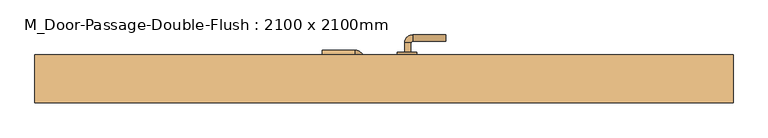
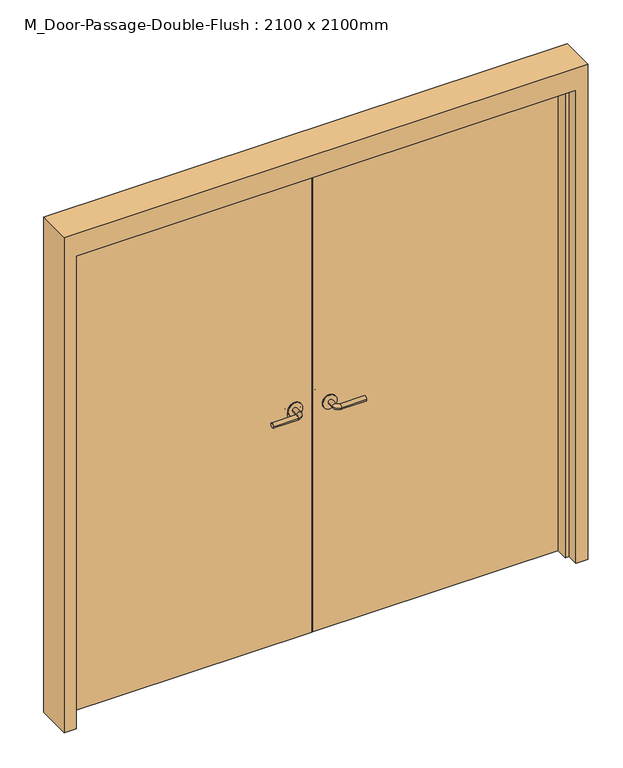
"""IFC4 building model written with IfcOpenShell, lengths in millimetres: door geometry, M_Door-Passage-Double-Flush : 2100 x 2100mm."""

from ifc_helpers import new_model, si_unit, point, frame, frame_2d, origin, origin_with_axes, place, context, project, spatial, polyline, circle_curve, ellipse_curve, trimmed, segment, composite_curve, outline, extrude, faceted_brep, source, transform, mapped, element, save
from ifc_brep_helpers import plane_surface, cylinder_surface, revolved_surface, advanced_brep


def m_door_passage_double_flush_2100_x_2100mm_eebec6e6(model_context):
    return source(origin(), model_context, "Body", "SolidModel", [
        advanced_brep(
        [(-65.009375, 78.35, 1016.0), (-85.009375, 78.35, 1016.0), (-65.009375, 48.35, 1016.0), (-85.009375, 48.35, 1016.0), (-90.009375, 43.35, 1016.0), (-90.009375, 23.35, 1016.0), (-195.009375, 23.35, 1016.0), (-195.009375, 43.35, 1016.0)],
        [
            (0, 1, circle_curve(frame((-75.009375, 78.35, 1016.0), z_axis=(0.0, 1.0, 0.0), x_axis=(-1.0, 0.0, 0.0)), 10.0)),
            (1, 0, circle_curve(frame((-75.009375, 78.35, 1016.0), z_axis=(0.0, 1.0, 0.0), x_axis=(-1.0, 0.0, 0.0)), 10.0)),
            (0, 2),
            (2, 3, circle_curve(frame((-75.009375, 48.35, 1016.0), z_axis=(0.0, 1.0, 0.0), x_axis=(-1.0, 0.0, 0.0)), 10.0)),
            (3, 1),
            (3, 2, circle_curve(frame((-75.009375, 48.35, 1016.0), z_axis=(0.0, 1.0, 0.0), x_axis=(-1.0, 0.0, 0.0)), 10.0)),
            (4, 3, circle_curve(frame((-90.009375, 48.35, 1016.0), z_axis=(0.0, 0.0, 1.0), x_axis=(1.0, 0.0, 0.0)), 5.0)),
            (2, 5, circle_curve(frame((-90.009375, 48.35, 1016.0), z_axis=(0.0, 0.0, -1.0), x_axis=(1.0, 0.0, 0.0)), 25.0)),
            (5, 4, circle_curve(frame((-90.009375, 33.35, 1016.0), z_axis=(1.0, 0.0, 0.0), x_axis=(0.0, 1.0, 0.0)), 10.0)),
            (4, 5, circle_curve(frame((-90.009375, 33.35, 1016.0), z_axis=(1.0, 0.0, 0.0), x_axis=(0.0, 1.0, 0.0)), 10.0)),
            (6, 7, circle_curve(frame((-195.009375, 33.35, 1016.0), z_axis=(-1.0, 0.0, 0.0), x_axis=(0.0, 1.0, 0.0)), 10.0)),
            (7, 6, circle_curve(frame((-195.009375, 33.35, 1016.0), z_axis=(-1.0, 0.0, 0.0), x_axis=(0.0, 1.0, 0.0)), 10.0)),
            (5, 6),
            (7, 4),
        ],
        [
            plane_surface(frame((-75.009375, 78.35, 1016.0), z_axis=(0.0, 1.0, 0.0), x_axis=(0.0, 0.0, 1.0))),
            cylinder_surface(frame((-75.009375, 78.35, 1016.0), z_axis=(0.0, 1.0, 0.0), x_axis=(-1.0, 0.0, 0.0)), 10.0),
            revolved_surface(trimmed(ellipse_curve(frame((-75.009375, 48.35, 1016.0), z_axis=(0.0, 1.0, 0.0), x_axis=(-1.0, 0.0, 0.0)), 10.0, 10.0), [point((-65.009375, 48.35, 1016.0))], [point((-85.009375, 48.35, 1016.0))], True, "CARTESIAN"), (-90.009375, 48.35, 1016.0), (0.0, 0.0, -1.0)),
            revolved_surface(trimmed(ellipse_curve(frame((-75.009375, 48.35, 1016.0), z_axis=(0.0, 1.0, 0.0), x_axis=(-1.0, 0.0, 0.0)), 10.0, 10.0), [point((-85.009375, 48.35, 1016.0))], [point((-65.009375, 48.35, 1016.0))], True, "CARTESIAN"), (-90.009375, 48.35, 1016.0), (0.0, 0.0, -1.0)),
            plane_surface(frame((-195.009375, 33.35, 1016.0), z_axis=(-1.0, 0.0, 0.0), x_axis=(0.0, 0.0, 1.0))),
            cylinder_surface(frame((-90.009375, 33.35, 1016.0), z_axis=(1.0, 0.0, 0.0), x_axis=(0.0, 1.0, 0.0)), 10.0),
        ],
        [
            (0, [[1, 2]]),
            (1, [[-1, 3, 4, 5]]),
            (1, [[-2, -5, 6, -3]]),
            (2, [[7, -4, 8, 9]]),
            (3, [[-8, -6, -7, 10]]),
            (4, [[11, 12]]),
            (5, [[-9, 13, -12, 14]]),
            (5, [[-10, -14, -11, -13]]),
        ],
    ),
        extrude(outline(composite_curve([segment(trimmed(circle_curve(frame_2d((1016.0, -72.509375)), 30.0), [point((1016.0, -42.509375))], [point((1016.0, -102.509375))], False, "CARTESIAN"), True, "CONTINUOUS"), segment(trimmed(circle_curve(frame_2d((1016.0, -72.509375)), 30.0), [point((1016.0, -102.509375))], [point((1016.0, -42.509375))], False, "CARTESIAN"), True, "CONTINUOUS")], self_intersect=False)), frame((0.0, 78.35, 0.0), z_axis=(0.0, 1.0, 0.0), x_axis=(0.0, 0.0, 1.0)), (0.0, 0.0, 1.0), 8.0),
        advanced_brep(
        [(-65.009375, 90.95, 1000.0), (-85.009375, 90.95, 1000.0), (-85.009375, 120.95, 1000.0), (-65.009375, 120.95, 1000.0), (-90.009375, 125.95, 1000.0), (-90.009375, 145.95, 1000.0), (-195.009375, 145.95, 1000.0), (-195.009375, 125.95, 1000.0)],
        [
            (0, 1, circle_curve(frame((-75.009375, 90.95, 1000.0), z_axis=(0.0, -1.0, 0.0), x_axis=(-1.0, 0.0, 0.0)), 10.0)),
            (1, 0, circle_curve(frame((-75.009375, 90.95, 1000.0), z_axis=(0.0, -1.0, 0.0), x_axis=(-1.0, 0.0, 0.0)), 10.0)),
            (1, 2),
            (2, 3, circle_curve(frame((-75.009375, 120.95, 1000.0), z_axis=(0.0, -1.0, 0.0), x_axis=(-1.0, 0.0, 0.0)), 10.0)),
            (3, 0),
            (3, 2, circle_curve(frame((-75.009375, 120.95, 1000.0), z_axis=(0.0, -1.0, 0.0), x_axis=(-1.0, 0.0, 0.0)), 10.0)),
            (4, 5, circle_curve(frame((-90.009375, 135.95, 1000.0), z_axis=(1.0, 0.0, 0.0), x_axis=(0.0, -1.0, 0.0)), 10.0)),
            (5, 3, circle_curve(frame((-90.009375, 120.95, 1000.0), z_axis=(0.0, 0.0, -1.0), x_axis=(1.0, 0.0, 0.0)), 25.0)),
            (2, 4, circle_curve(frame((-90.009375, 120.95, 1000.0), z_axis=(0.0, 0.0, 1.0), x_axis=(1.0, 0.0, 0.0)), 5.0)),
            (5, 4, circle_curve(frame((-90.009375, 135.95, 1000.0), z_axis=(1.0, 0.0, 0.0), x_axis=(0.0, -1.0, 0.0)), 10.0)),
            (6, 7, circle_curve(frame((-195.009375, 135.95, 1000.0), z_axis=(-1.0, 0.0, 0.0), x_axis=(0.0, -1.0, 0.0)), 10.0)),
            (7, 6, circle_curve(frame((-195.009375, 135.95, 1000.0), z_axis=(-1.0, 0.0, 0.0), x_axis=(0.0, -1.0, 0.0)), 10.0)),
            (4, 7),
            (6, 5),
        ],
        [
            plane_surface(frame((-75.009375, 90.95, 1000.0), z_axis=(0.0, -1.0, 0.0), x_axis=(0.0, 0.0, 1.0))),
            cylinder_surface(frame((-75.009375, 90.95, 1000.0), z_axis=(0.0, -1.0, 0.0), x_axis=(-1.0, 0.0, 0.0)), 10.0),
            revolved_surface(trimmed(ellipse_curve(frame((-75.009375, 120.95, 1000.0), z_axis=(0.0, 1.0, 0.0), x_axis=(-1.0, 0.0, 0.0)), 10.0, 10.0), [point((-65.009375, 120.95, 1000.0))], [point((-85.009375, 120.95, 1000.0))], True, "CARTESIAN"), (-90.009375, 120.95, 1000.0), (0.0, 0.0, -1.0)),
            revolved_surface(trimmed(ellipse_curve(frame((-75.009375, 120.95, 1000.0), z_axis=(0.0, 1.0, 0.0), x_axis=(-1.0, 0.0, 0.0)), 10.0, 10.0), [point((-85.009375, 120.95, 1000.0))], [point((-65.009375, 120.95, 1000.0))], True, "CARTESIAN"), (-90.009375, 120.95, 1000.0), (0.0, 0.0, -1.0)),
            plane_surface(frame((-195.009375, 135.95, 1000.0), z_axis=(-1.0, 0.0, 0.0), x_axis=(0.0, 0.0, 1.0))),
            cylinder_surface(frame((-90.009375, 135.95, 1000.0), z_axis=(1.0, 0.0, 0.0), x_axis=(0.0, -1.0, 0.0)), 10.0),
        ],
        [
            (0, [[1, 2]]),
            (1, [[3, 4, 5, -2]]),
            (1, [[-5, 6, -3, -1]]),
            (2, [[7, 8, -4, 9]]),
            (3, [[10, -9, -6, -8]]),
            (4, [[11, 12]]),
            (5, [[13, -11, 14, -7]]),
            (5, [[-14, -12, -13, -10]]),
        ],
    ),
        extrude(outline(composite_curve([segment(trimmed(circle_curve(frame_2d((1000.0, -72.509375)), 30.0), [point((1000.0, -42.509375))], [point((1000.0, -102.509375))], False, "CARTESIAN"), True, "CONTINUOUS"), segment(trimmed(circle_curve(frame_2d((1000.0, -72.509375)), 30.0), [point((1000.0, -102.509375))], [point((1000.0, -42.509375))], False, "CARTESIAN"), True, "CONTINUOUS")], self_intersect=False)), frame((0.0, 82.95, 0.0), z_axis=(0.0, 1.0, 0.0), x_axis=(0.0, 0.0, 1.0)), (0.0, 0.0, 1.0), 8.0),
        advanced_brep(
        [(65.009375, 78.35, 1000.0), (85.009375, 78.35, 1000.0), (85.009375, 48.35, 1000.0), (65.009375, 48.35, 1000.0), (90.009375, 43.35, 1000.0), (90.009375, 23.35, 1000.0), (195.009375, 23.35, 1000.0), (195.009375, 43.35, 1000.0)],
        [
            (0, 1, circle_curve(frame((75.009375, 78.35, 1000.0), z_axis=(0.0, 1.0, 0.0), x_axis=(1.0, 0.0, 0.0)), 10.0)),
            (1, 0, circle_curve(frame((75.009375, 78.35, 1000.0), z_axis=(0.0, 1.0, 0.0), x_axis=(1.0, 0.0, 0.0)), 10.0)),
            (1, 2),
            (2, 3, circle_curve(frame((75.009375, 48.35, 1000.0), z_axis=(0.0, 1.0, 0.0), x_axis=(1.0, 0.0, 0.0)), 10.0)),
            (3, 0),
            (3, 2, circle_curve(frame((75.009375, 48.35, 1000.0), z_axis=(0.0, 1.0, 0.0), x_axis=(1.0, 0.0, 0.0)), 10.0)),
            (4, 5, circle_curve(frame((90.009375, 33.35, 1000.0), z_axis=(-1.0, 0.0, 0.0), x_axis=(0.0, 1.0, 0.0)), 10.0)),
            (5, 3, circle_curve(frame((90.009375, 48.35, 1000.0), z_axis=(0.0, 0.0, -1.0), x_axis=(-1.0, 0.0, 0.0)), 25.0)),
            (2, 4, circle_curve(frame((90.009375, 48.35, 1000.0), z_axis=(0.0, 0.0, 1.0), x_axis=(-1.0, 0.0, 0.0)), 5.0)),
            (5, 4, circle_curve(frame((90.009375, 33.35, 1000.0), z_axis=(-1.0, 0.0, 0.0), x_axis=(0.0, 1.0, 0.0)), 10.0)),
            (6, 7, circle_curve(frame((195.009375, 33.35, 1000.0), z_axis=(1.0, 0.0, 0.0), x_axis=(0.0, 1.0, 0.0)), 10.0)),
            (7, 6, circle_curve(frame((195.009375, 33.35, 1000.0), z_axis=(1.0, 0.0, 0.0), x_axis=(0.0, 1.0, 0.0)), 10.0)),
            (4, 7),
            (6, 5),
        ],
        [
            plane_surface(frame((75.009375, 78.35, 1000.0), z_axis=(0.0, 1.0, 0.0), x_axis=(0.0, 0.0, 1.0))),
            cylinder_surface(frame((75.009375, 78.35, 1000.0), z_axis=(0.0, 1.0, 0.0), x_axis=(1.0, 0.0, 0.0)), 10.0),
            revolved_surface(trimmed(ellipse_curve(frame((75.009375, 48.35, 1000.0), z_axis=(0.0, -1.0, 0.0), x_axis=(1.0, 0.0, 0.0)), 10.0, 10.0), [point((65.009375, 48.35, 1000.0))], [point((85.009375, 48.35, 1000.0))], True, "CARTESIAN"), (90.009375, 48.35, 1000.0), (0.0, 0.0, -1.0)),
            revolved_surface(trimmed(ellipse_curve(frame((75.009375, 48.35, 1000.0), z_axis=(0.0, -1.0, 0.0), x_axis=(1.0, 0.0, 0.0)), 10.0, 10.0), [point((85.009375, 48.35, 1000.0))], [point((65.009375, 48.35, 1000.0))], True, "CARTESIAN"), (90.009375, 48.35, 1000.0), (0.0, 0.0, -1.0)),
            plane_surface(frame((195.009375, 33.35, 1000.0), z_axis=(1.0, 0.0, 0.0), x_axis=(0.0, 0.0, 1.0))),
            cylinder_surface(frame((90.009375, 33.35, 1000.0), z_axis=(-1.0, 0.0, 0.0), x_axis=(0.0, 1.0, 0.0)), 10.0),
        ],
        [
            (0, [[1, 2]]),
            (1, [[3, 4, 5, -2]]),
            (1, [[-5, 6, -3, -1]]),
            (2, [[7, 8, -4, 9]]),
            (3, [[10, -9, -6, -8]]),
            (4, [[11, 12]]),
            (5, [[13, -11, 14, -7]]),
            (5, [[-14, -12, -13, -10]]),
        ],
    ),
        extrude(outline(composite_curve([segment(trimmed(circle_curve(frame_2d((1000.0, 72.509375)), 30.0), [point((1000.0, 42.509375))], [point((1000.0, 102.509375))], False, "CARTESIAN"), True, "CONTINUOUS"), segment(trimmed(circle_curve(frame_2d((1000.0, 72.509375)), 30.0), [point((1000.0, 102.509375))], [point((1000.0, 42.509375))], False, "CARTESIAN"), True, "CONTINUOUS")], self_intersect=False)), frame((0.0, 78.35, 0.0), z_axis=(0.0, 1.0, 0.0), x_axis=(0.0, 0.0, 1.0)), (0.0, 0.0, 1.0), 8.0),
        advanced_brep(
        [(65.009375, 139.35, 1000.0), (85.009375, 139.35, 1000.0), (65.009375, 169.35, 1000.0), (85.009375, 169.35, 1000.0), (90.009375, 174.35, 1000.0), (90.009375, 194.35, 1000.0), (195.009375, 194.35, 1000.0), (195.009375, 174.35, 1000.0)],
        [
            (0, 1, circle_curve(frame((75.009375, 139.35, 1000.0), z_axis=(0.0, -1.0, 0.0), x_axis=(1.0, 0.0, 0.0)), 10.0)),
            (1, 0, circle_curve(frame((75.009375, 139.35, 1000.0), z_axis=(0.0, -1.0, 0.0), x_axis=(1.0, 0.0, 0.0)), 10.0)),
            (0, 2),
            (2, 3, circle_curve(frame((75.009375, 169.35, 1000.0), z_axis=(0.0, -1.0, 0.0), x_axis=(1.0, 0.0, 0.0)), 10.0)),
            (3, 1),
            (3, 2, circle_curve(frame((75.009375, 169.35, 1000.0), z_axis=(0.0, -1.0, 0.0), x_axis=(1.0, 0.0, 0.0)), 10.0)),
            (4, 3, circle_curve(frame((90.009375, 169.35, 1000.0), z_axis=(0.0, 0.0, 1.0), x_axis=(-1.0, 0.0, 0.0)), 5.0)),
            (2, 5, circle_curve(frame((90.009375, 169.35, 1000.0), z_axis=(0.0, 0.0, -1.0), x_axis=(-1.0, 0.0, 0.0)), 25.0)),
            (5, 4, circle_curve(frame((90.009375, 184.35, 1000.0), z_axis=(-1.0, 0.0, 0.0), x_axis=(0.0, -1.0, 0.0)), 10.0)),
            (4, 5, circle_curve(frame((90.009375, 184.35, 1000.0), z_axis=(-1.0, 0.0, 0.0), x_axis=(0.0, -1.0, 0.0)), 10.0)),
            (6, 7, circle_curve(frame((195.009375, 184.35, 1000.0), z_axis=(1.0, 0.0, 0.0), x_axis=(0.0, -1.0, 0.0)), 10.0)),
            (7, 6, circle_curve(frame((195.009375, 184.35, 1000.0), z_axis=(1.0, 0.0, 0.0), x_axis=(0.0, -1.0, 0.0)), 10.0)),
            (5, 6),
            (7, 4),
        ],
        [
            plane_surface(frame((75.009375, 139.35, 1000.0), z_axis=(0.0, -1.0, 0.0), x_axis=(0.0, 0.0, 1.0))),
            cylinder_surface(frame((75.009375, 139.35, 1000.0), z_axis=(0.0, -1.0, 0.0), x_axis=(1.0, 0.0, 0.0)), 10.0),
            revolved_surface(trimmed(ellipse_curve(frame((75.009375, 169.35, 1000.0), z_axis=(0.0, -1.0, 0.0), x_axis=(1.0, 0.0, 0.0)), 10.0, 10.0), [point((65.009375, 169.35, 1000.0))], [point((85.009375, 169.35, 1000.0))], True, "CARTESIAN"), (90.009375, 169.35, 1000.0), (0.0, 0.0, -1.0)),
            revolved_surface(trimmed(ellipse_curve(frame((75.009375, 169.35, 1000.0), z_axis=(0.0, -1.0, 0.0), x_axis=(1.0, 0.0, 0.0)), 10.0, 10.0), [point((85.009375, 169.35, 1000.0))], [point((65.009375, 169.35, 1000.0))], True, "CARTESIAN"), (90.009375, 169.35, 1000.0), (0.0, 0.0, -1.0)),
            plane_surface(frame((195.009375, 184.35, 1000.0), z_axis=(1.0, 0.0, 0.0), x_axis=(0.0, 0.0, 1.0))),
            cylinder_surface(frame((90.009375, 184.35, 1000.0), z_axis=(-1.0, 0.0, 0.0), x_axis=(0.0, -1.0, 0.0)), 10.0),
        ],
        [
            (0, [[1, 2]]),
            (1, [[-1, 3, 4, 5]]),
            (1, [[-2, -5, 6, -3]]),
            (2, [[7, -4, 8, 9]]),
            (3, [[-8, -6, -7, 10]]),
            (4, [[11, 12]]),
            (5, [[-9, 13, -12, 14]]),
            (5, [[-10, -14, -11, -13]]),
        ],
    ),
        extrude(outline(composite_curve([segment(trimmed(circle_curve(frame_2d((1000.0, 72.509375)), 30.0), [point((1000.0, 42.509375))], [point((1000.0, 102.509375))], False, "CARTESIAN"), True, "CONTINUOUS"), segment(trimmed(circle_curve(frame_2d((1000.0, 72.509375)), 30.0), [point((1000.0, 102.509375))], [point((1000.0, 42.509375))], False, "CARTESIAN"), True, "CONTINUOUS")], self_intersect=False)), frame((0.0, 131.35, 0.0), z_axis=(0.0, 1.0, 0.0), x_axis=(0.0, 0.0, 1.0)), (0.0, 0.0, 1.0), 8.0),
        faceted_brep([(1050.0, 81.5875, 0.0), (1050.0, 131.35, 0.0), (1100.0, 131.35, 0.0), (1100.0, -18.65, 0.0), (1050.0, -18.65, 0.0), (1050.0, 30.5625, 0.0), (1034.125, 30.5625, 0.0), (1034.125, 81.5875, 0.0), (1050.0, 81.5875, 2100.0), (1050.0, 131.35, 2100.0), (-1050.0, 131.35, 2100.0), (-1050.0, 131.35, 0.0), (-1100.0, 131.35, 0.0), (-1100.0, 131.35, 2200.0), (1100.0, 131.35, 2200.0), (1100.0, -18.65, 2200.0), (-1100.0, -18.65, 2200.0), (-1100.0, -18.65, 0.0), (-1050.0, -18.65, 0.0), (-1050.0, -18.65, 2100.0), (1050.0, -18.65, 2100.0), (1050.0, 30.5625, 2100.0), (-1050.0, 30.5625, 2100.0), (-1050.0, 30.5625, 0.0), (-1034.125, 30.5625, 0.0), (-1034.125, 30.5625, 2084.125), (1034.125, 30.5625, 2084.125), (1034.125, 81.5875, 2084.125), (-1034.125, 81.5875, 2084.125), (-1034.125, 81.5875, 0.0), (-1050.0, 81.5875, 0.0), (-1050.0, 81.5875, 2100.0)], [[[0, 1, 2, 3, 4, 5, 6, 7]], [[1, 0, 8, 9]], [[2, 1, 9, 10, 11, 12, 13, 14]], [[3, 2, 14, 15]], [[4, 3, 15, 16, 17, 18, 19, 20]], [[5, 4, 20, 21]], [[6, 5, 21, 22, 23, 24, 25, 26]], [[7, 6, 26, 27]], [[0, 7, 27, 28, 29, 30, 31, 8]], [[9, 8, 31, 10]], [[20, 19, 22, 21]], [[26, 25, 28, 27]], [[12, 11, 30, 29, 24, 23, 18, 17]], [[11, 10, 31, 30]], [[13, 12, 17, 16]], [[19, 18, 23, 22]], [[25, 24, 29, 28]], [[15, 14, 13, 16]]]),
        extrude(outline(polyline([(1050.0, 82.95), (1.5875, 82.95), (1.5875, 86.35), (1050.0, 86.35), (1050.0, 82.95)])), origin_with_axes(), (0.0, 0.0, 1.0), 2100.0),
        extrude(outline(polyline([(-1.5875, 82.95), (-1050.0, 82.95), (-1050.0, 86.35), (-1.5875, 86.35), (-1.5875, 82.95)])), origin_with_axes(), (0.0, 0.0, 1.0), 2100.0),
    ])


if __name__ == "__main__":
    model = new_model("IFC4")
    model_context = context("Model", 3, world=origin())
    ifc_project = project(units=[si_unit("LENGTHUNIT", "METRE", prefix="MILLI")], contexts=[model_context])
    site = spatial("IfcSite", under=ifc_project)
    building = spatial("IfcBuilding", under=site)
    placement = place(None, origin())
    m_door_passage_double_flush_2100_x_2100mm_shape = m_door_passage_double_flush_2100_x_2100mm_eebec6e6(model_context)
    element("IfcDoor", 1, ObjectType="M_Door-Passage-Double-Flush : 2100 x 2100mm", at=placement, inside=building, context=model_context, shape_type="MappedRepresentation", body=[
        mapped(m_door_passage_double_flush_2100_x_2100mm_shape, transform((0.0, 0.0, 0.0), x_axis=(1.0, 0.0, 0.0), y_axis=(0.0, 1.0, 0.0), z_axis=(0.0, 0.0, 1.0))),
    ])
    save(model, "model.ifc")

# Revit data of these elements
# Type "M_Door-Passage-Double-Flush : 2100 x 2100mm"
#   Type Mark = "40"
#   Assembly Code = "B2030200"
#   Analytic Construction = "Metal"
#   Thickness = 45 mm
#   Thermal Resistance (R) = 0.270118 (m²·K)/W
#   Swing Angle [instance default] = 90.00°
#   Strike Height = 1000 mm
#   SinglePanelWidth = 1050 mm
#   Rough Width [instance default] = 2200 mm
#   Rough Height [instance default] = 2200 mm
#   MFOpeningHeight [instance default] = 100 mm
#   MFOpeningWidth [instance default] = 100 mm
#   Inset Calculate [instance default] = 105 mm
#   Masonry Inset [instance default] = 25 mm
#   Height = 2100 mm
#   Width = 2100 mm
#   Heat Transfer Coefficient (U) = 3.70223 W/(m²·K)
#   Masonry Frame Depth = 150 mm
#   Masonry Frame [instance default] = yes
#   Function = 1
#   Dry Wall Frame [instance default] = no
#   Panel Material = Metal Door - Brindle
#   Frame Material = Metal - Painted - Grey
#   Door Handle Material = Aluminum
#   Visual Light Transmittance = 0
#   Solar Heat Gain Coefficient = 0
#   Wall Closure = (empty or 0)
# Element 1 (IfcDoor, "M_Door-Passage-Double-Flush : 2100 x 2100mm")
#   Materials on its faces: "Aluminum", "Metal - Painted - Grey", "Metal Door - Brindle"
# Materials
#   "Metal Door - Brindle": class "Paint", colour RGB 164 133 98, transparency 0
#   "Metal - Painted - Grey": class "Paint", colour RGB 104 104 104, transparency 0
#   "Aluminum": class "Metal", colour RGB 244 244 244, transparency 0, Description = "Aluminum 6061", Cost = 0
